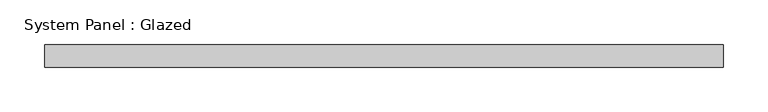
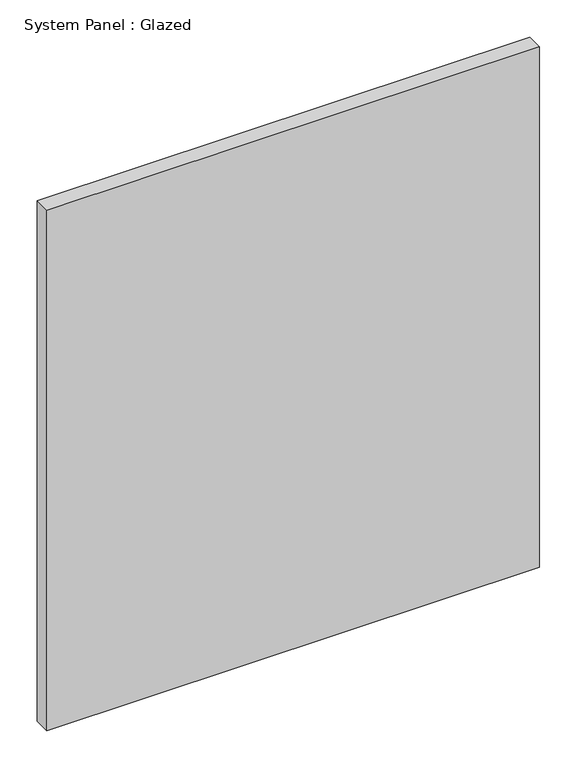
"""IFC4 building model written with IfcOpenShell, lengths in millimetres: plate geometry, System Panel : Glazed."""

import ifcopenshell
import ifcopenshell.guid

model = None  # the IFC model being written
_history = None  # IfcOwnerHistory: only IFC2X3 demands one
_inside = {}  # id of a spatial element -> (the spatial element, [elements in it])
_under = {}  # id of a project, library or spatial element -> (it, [spatial elements below it])
_declared = {}  # id of a project -> (the project, [libraries it declares])
_typed = {}  # id of a type object -> (the type object, [elements of that type])
_made_of = {}  # id of a material, layer set ... -> (it, [elements and type objects made of it])


def new_model(schema):
    """Start an empty IFC model of exactly this schema.

    Asked for "IFC4X3", IfcOpenShell would pick the latest addendum, in which some entities
    have other attributes; the version numbers below select the first issue.
    IFC2X3 requires an IfcOwnerHistory on every rooted entity: one is made here for all.
    """
    global model, _history
    if schema == "IFC4X3":
        model = ifcopenshell.file(schema_version=(4, 3, 0, 0))
    else:
        model = ifcopenshell.file(schema=schema)
    _inside.clear()
    _under.clear()
    _declared.clear()
    _typed.clear()
    _made_of.clear()
    _history = None
    if model.schema == "IFC2X3":
        org = make("IfcOrganization", Name="unknown")
        user = make(
            "IfcPersonAndOrganization",
            ThePerson=make("IfcPerson", FamilyName="unknown"),
            TheOrganization=org,
        )
        app = make(
            "IfcApplication",
            ApplicationDeveloper=org,
            Version="unknown",
            ApplicationFullName="unknown",
            ApplicationIdentifier="unknown",
        )
        _history = make(
            "IfcOwnerHistory",
            OwningUser=user,
            OwningApplication=app,
            ChangeAction="ADDED",
            CreationDate=0,
        )
    return model


def make(cls, **values):
    """One entity of the class cls with the attributes given. An attribute that is None is left unset."""
    return model.create_entity(
        cls, **{name: value for name, value in values.items() if value is not None}
    )


def rooted(cls, **values):
    """An entity with a GlobalId (a new one), such as an element, a storey or a relation."""
    return make(cls, GlobalId=ifcopenshell.guid.new(), OwnerHistory=_history, **values)


def si_unit(unit_type, name, prefix=None):
    """IfcSIUnit, for example si_unit("LENGTHUNIT", "METRE", prefix="MILLI")."""
    return make("IfcSIUnit", UnitType=unit_type, Prefix=prefix, Name=name)


def assignment(units):
    """IfcUnitAssignment: the units of a project."""
    return None if units is None else make("IfcUnitAssignment", Units=units)


def point(xyz):
    """IfcCartesianPoint."""
    return None if xyz is None else make("IfcCartesianPoint", Coordinates=xyz)


def direction(xyz):
    """IfcDirection."""
    return None if xyz is None else make("IfcDirection", DirectionRatios=xyz)


def frame(location, z_axis=None, x_axis=None):
    """IfcAxis2Placement3D, a coordinate frame: its origin and axes. An axis left out is left unset."""
    return make(
        "IfcAxis2Placement3D",
        Location=point(location),
        Axis=direction(z_axis),
        RefDirection=direction(x_axis),
    )


def origin():
    """The frame at (0, 0, 0) with its axes left unset."""
    return frame((0.0, 0.0, 0.0))


def origin_with_axes():
    """The frame at (0, 0, 0) with the z axis (0, 0, 1) and the x axis (1, 0, 0) written out."""
    return frame((0.0, 0.0, 0.0), z_axis=(0.0, 0.0, 1.0), x_axis=(1.0, 0.0, 0.0))


def place(relative_to, where):
    """IfcLocalPlacement: puts the frame where relative to a parent placement (None: the world)."""
    return make(
        "IfcLocalPlacement", PlacementRelTo=relative_to, RelativePlacement=where
    )


def context(
    kind, dimensions, precision=None, world=None, true_north=None, identifier=None
):
    """IfcGeometricRepresentationContext, for example the 3D "Model" context."""
    return make(
        "IfcGeometricRepresentationContext",
        ContextIdentifier=identifier,
        ContextType=kind,
        CoordinateSpaceDimension=dimensions,
        Precision=precision,
        WorldCoordinateSystem=world,
        TrueNorth=true_north,
    )


def project(units=None, contexts=None):
    """IfcProject with its units and contexts."""
    return rooted(
        "IfcProject",
        Name="project",
        RepresentationContexts=contexts,
        UnitsInContext=assignment(units),
    )


def spatial(cls, under=None, at=None, **own):
    """A site, building, storey or space (cls), placed at a placement, below another one or the project."""
    s = rooted(cls, ObjectPlacement=at, **own)
    if under is not None:
        _under.setdefault(under.id(), (under, []))[1].append(s)
    return s


def polyline(points):
    """IfcPolyline through the points."""
    return make("IfcPolyline", Points=[point(p) for p in points])


def outline(outer, holes=None, kind="AREA"):
    """IfcArbitraryClosedProfileDef: a profile drawn as a closed curve; with holes, ...WithVoids."""
    if holes is None:
        return make("IfcArbitraryClosedProfileDef", ProfileType=kind, OuterCurve=outer)
    return make(
        "IfcArbitraryProfileDefWithVoids",
        ProfileType=kind,
        OuterCurve=outer,
        InnerCurves=holes,
    )


def extrude(swept, where, along, depth):
    """IfcExtrudedAreaSolid: the profile swept, set in the frame where, extruded along a direction by depth."""
    return make(
        "IfcExtrudedAreaSolid",
        SweptArea=swept,
        Position=where,
        ExtrudedDirection=direction(along),
        Depth=depth,
    )


def shape(context_of_items, identifier, shape_type, items):
    """IfcShapeRepresentation: the items that make up one representation, for example the "Body"."""
    return make(
        "IfcShapeRepresentation",
        ContextOfItems=context_of_items,
        RepresentationIdentifier=identifier,
        RepresentationType=shape_type,
        Items=items,
    )


def source(mapping_origin, context_of_items, identifier, shape_type, items):
    """IfcRepresentationMap: a shape defined once, which mapped items show again and again."""
    return make(
        "IfcRepresentationMap",
        MappingOrigin=mapping_origin,
        MappedRepresentation=shape(context_of_items, identifier, shape_type, items),
    )


def transform(
    local_origin,
    x_axis=None,
    y_axis=None,
    z_axis=None,
    scale=None,
    scale2=None,
    scale3=None,
    uniform=True,
):
    """IfcCartesianTransformationOperator3D, or its non-uniform kind. x_axis, y_axis, z_axis: its Axis1, 2, 3."""
    if uniform:
        return make(
            "IfcCartesianTransformationOperator3D",
            Axis1=direction(x_axis),
            Axis2=direction(y_axis),
            LocalOrigin=point(local_origin),
            Scale=scale,
            Axis3=direction(z_axis),
        )
    return make(
        "IfcCartesianTransformationOperator3DnonUniform",
        Axis1=direction(x_axis),
        Axis2=direction(y_axis),
        LocalOrigin=point(local_origin),
        Scale=scale,
        Axis3=direction(z_axis),
        Scale2=scale2,
        Scale3=scale3,
    )


def mapped(mapping_source, mapping_target):
    """IfcMappedItem: shows the shape of a source again, moved by a transform."""
    return make(
        "IfcMappedItem", MappingSource=mapping_source, MappingTarget=mapping_target
    )


def made_of(thing, what):
    """Note that an element or type object is made of a material, layer set ...; save() writes the relation."""
    if what is not None:
        _made_of.setdefault(what.id(), (what, []))[1].append(thing)
    return thing


def element(
    cls,
    number,
    at=None,
    inside=None,
    cuts=None,
    type_object=None,
    material=None,
    context=None,
    identifier="Body",
    shape_type=None,
    held_by="IfcProductDefinitionShape",
    body=None,
    shapes=None,
    **own,
):
    """One element of the class cls, such as IfcWall. Its Tag is "e" and its number.

    at: its placement. inside: the storey or other place that contains it. cuts: it is an
    opening in that element (IfcRelVoidsElement). A single representation is given by context,
    identifier, shape_type and body (its items); several are given by shapes. held_by: the class
    of the entity that holds the representations. save() writes the other relations.
    """
    e = rooted(cls, Tag="e%d" % number, ObjectPlacement=at, **own)
    if body is not None:
        shapes = [shape(context, identifier, shape_type, body)]
    if shapes is not None:
        e.Representation = make(held_by, Representations=shapes)
    if inside is not None:
        _inside.setdefault(inside.id(), (inside, []))[1].append(e)
    if cuts is not None:
        rooted(
            "IfcRelVoidsElement", RelatingBuildingElement=cuts, RelatedOpeningElement=e
        )
    if type_object is not None:
        _typed.setdefault(type_object.id(), (type_object, []))[1].append(e)
    return made_of(e, material)


def aggregate(whole, parts):
    """IfcRelAggregates: a whole, such as a stair, and the parts it consists of."""
    return rooted("IfcRelAggregates", RelatingObject=whole, RelatedObjects=parts)


def save(model, path):
    """Write the relations noted so far, then the file.

    IfcRelAggregates (storeys below a building ...), IfcRelContainedInSpatialStructure (elements
    in a storey), IfcRelDefinesByType, IfcRelAssociatesMaterial and IfcRelDeclares: one each for
    every whole, place, type object, material and project.
    """
    for whole, parts in _under.values():
        aggregate(whole, parts)
    for where, things in _inside.values():
        rooted(
            "IfcRelContainedInSpatialStructure",
            RelatedElements=things,
            RelatingStructure=where,
        )
    for kind, things in _typed.values():
        rooted("IfcRelDefinesByType", RelatedObjects=things, RelatingType=kind)
    for what, things in _made_of.values():
        rooted("IfcRelAssociatesMaterial", RelatedObjects=things, RelatingMaterial=what)
    for by, libraries in _declared.values():
        rooted("IfcRelDeclares", RelatingContext=by, RelatedDefinitions=libraries)
    model.write(path)


def system_panel_glazed_4fa5cbd7(model_context):
    return source(origin(), model_context, "Body", "SweptSolid", [
        extrude(outline(polyline([(381.0, 19.05), (-381.0, 19.05), (-381.0, 44.45), (381.0, 44.45), (381.0, 19.05)])), origin_with_axes(), (0.0, 0.0, 1.0), 850.9),
    ])


if __name__ == "__main__":
    model = new_model("IFC4")
    model_context = context("Model", 3, world=origin())
    ifc_project = project(units=[si_unit("LENGTHUNIT", "METRE", prefix="MILLI")], contexts=[model_context])
    site = spatial("IfcSite", under=ifc_project)
    building = spatial("IfcBuilding", under=site)
    placement = place(None, origin())
    system_panel_glazed_shape = system_panel_glazed_4fa5cbd7(model_context)
    element("IfcPlate", 1, ObjectType="System Panel : Glazed", at=placement, inside=building, context=model_context, shape_type="MappedRepresentation", body=[
        mapped(system_panel_glazed_shape, transform((0.0, 0.0, 0.0), x_axis=(1.0, 0.0, 0.0), y_axis=(0.0, 1.0, 0.0), z_axis=(0.0, 0.0, 1.0))),
    ])
    save(model, "model.ifc")

# Revit data of these elements
# Type "System Panel : Glazed"
#   Construction Type Id = "GSP4R"
#   Analytic Construction = "1/8 in Pilkington single glazing"
#   Visual Light Transmittance = 0.9
#   Solar Heat Gain Coefficient = 0.86
#   Heat Transfer Coefficient (U) = 1.18115 BTU/(h·ft²·°F)
#   Define Thermal Properties by = 1
# Element 1 (IfcPlate, "System Panel : Glazed")
#   Materials on its faces: "Glass"
# Materials
#   "Glass": class "Glass", colour RGB 0 128 192, transparency 0.75, Description = "Soda Lime Glass", Cost = 0
